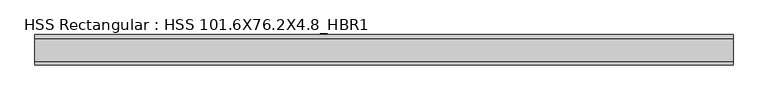
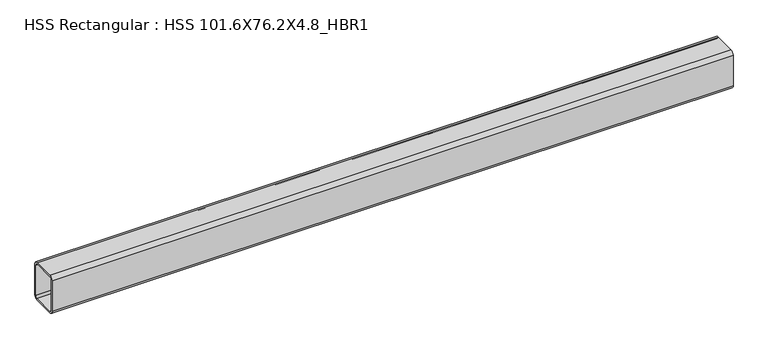
"""IFC4 building model written with IfcOpenShell, lengths in millimetres: beam geometry, HSS Rectangular : HSS 101.6X76.2X4.8_HBR1."""

from ifc_helpers import new_model, si_unit, point, frame, frame_2d, origin, place, context, project, spatial, polyline, circle_curve, trimmed, segment, composite_curve, outline, extrude, source, transform, mapped, element, save


def hss_rectangular_hss_101_6x76_2x4_8_hbr1_9ee25929(model_context):
    return source(origin(), model_context, "Body", "SweptSolid", [
        extrude(outline(composite_curve([segment(polyline([(38.1, 41.275), (38.1, -41.275)]), True, "CONTINUOUS"), segment(trimmed(circle_curve(frame_2d((28.575, -41.275)), 9.525), [point((38.1, -41.275))], [point((28.575, -50.8))], False, "CARTESIAN"), True, "CONTINUOUS"), segment(polyline([(28.575, -50.8), (-28.575, -50.8)]), True, "CONTINUOUS"), segment(trimmed(circle_curve(frame_2d((-28.575, -41.275)), 9.525), [point((-28.575, -50.8))], [point((-38.1, -41.275))], False, "CARTESIAN"), True, "CONTINUOUS"), segment(polyline([(-38.1, -41.275), (-38.1, 41.275)]), True, "CONTINUOUS"), segment(trimmed(circle_curve(frame_2d((-28.575, 41.275)), 9.525), [point((-38.1, 41.275))], [point((-28.575, 50.8))], False, "CARTESIAN"), True, "CONTINUOUS"), segment(polyline([(-28.575, 50.8), (28.575, 50.8)]), True, "CONTINUOUS"), segment(trimmed(circle_curve(frame_2d((28.575, 41.275)), 9.525), [point((28.575, 50.8))], [point((38.1, 41.275))], False, "CARTESIAN"), True, "CONTINUOUS")], self_intersect=False), holes=[composite_curve([segment(trimmed(circle_curve(frame_2d((-28.575, 41.275)), 4.7625), [point((-28.575, 46.0375))], [point((-33.3375, 41.275))], True, "CARTESIAN"), True, "CONTINUOUS"), segment(polyline([(-33.3375, 41.275), (-33.3375, -41.275)]), True, "CONTINUOUS"), segment(trimmed(circle_curve(frame_2d((-28.575, -41.275)), 4.7625), [point((-33.3375, -41.275))], [point((-28.575, -46.0375))], True, "CARTESIAN"), True, "CONTINUOUS"), segment(polyline([(-28.575, -46.0375), (28.575, -46.0375)]), True, "CONTINUOUS"), segment(trimmed(circle_curve(frame_2d((28.575, -41.275)), 4.7625), [point((28.575, -46.0375))], [point((33.3375, -41.275))], True, "CARTESIAN"), True, "CONTINUOUS"), segment(polyline([(33.3375, -41.275), (33.3375, 41.275)]), True, "CONTINUOUS"), segment(trimmed(circle_curve(frame_2d((28.575, 41.275)), 4.7625), [point((33.3375, 41.275))], [point((28.575, 46.0375))], True, "CARTESIAN"), True, "CONTINUOUS"), segment(polyline([(28.575, 46.0375), (-28.575, 46.0375)]), True, "CONTINUOUS")], self_intersect=False)]), frame((-850.0, 0.0, 0.0), z_axis=(1.0, 0.0, 0.0), x_axis=(0.0, 1.0, 0.0)), (0.0, 0.0, 1.0), 1747.4492101),
    ])


if __name__ == "__main__":
    model = new_model("IFC4")
    model_context = context("Model", 3, world=origin())
    ifc_project = project(units=[si_unit("LENGTHUNIT", "METRE", prefix="MILLI")], contexts=[model_context])
    site = spatial("IfcSite", under=ifc_project)
    building = spatial("IfcBuilding", under=site)
    placement = place(None, origin())
    hss_rectangular_hss_101_6x76_2x4_8_hbr1_shape = hss_rectangular_hss_101_6x76_2x4_8_hbr1_9ee25929(model_context)
    element("IfcBeam", 1, ObjectType="HSS Rectangular : HSS 101.6X76.2X4.8_HBR1", at=placement, inside=building, context=model_context, shape_type="MappedRepresentation", body=[
        mapped(hss_rectangular_hss_101_6x76_2x4_8_hbr1_shape, transform((0.0, 0.0, 0.0), x_axis=(1.0, 0.0, 0.0), y_axis=(0.0, 1.0, 0.0), z_axis=(0.0, 0.0, 1.0))),
    ])
    save(model, "model.ifc")

# Revit data of these elements
# Type "HSS Rectangular : HSS 101.6X76.2X4.8_HBR1"
#   Section Name Key = "HSS 4X3X3/16"
#   Assembly Code = "B10"
#   Width = 7.62 cm
#   Wall Nominal Thickness = 0.4763 cm
#   Wall Design Thickness = 0.442 cm
#   Torsional Moment of Inertia = 260.561 cm⁴
#   Torsional Modulus = 61.2876 cm³
#   Section Area = 14.4516 cm²
#   Plastic Modulus weak axis = 40.3122 cm³
#   Plastic Modulus strong axis = 49.1612 cm³
#   Perimeter = 0.881482 m²/m
#   Outer Fillet = 0.9525 cm
#   Nominal Weight = 12.1285 kgf/m
#   Moment of Inertia weak axis = 131.529 cm⁴
#   Moment of Inertia strong axis = 205.202 cm⁴
#   Inner Fillet = 0.4763 cm
#   Height = 10.16 cm
#   Elastic Modulus weak axis = 34.4128 cm³
#   Elastic Modulus strong axis = 40.476 cm³
#   Centroid Vertical = 5.08 cm
#   Centroid Horizontal = 3.81 cm
#   Length [instance default] = 1524 mm
#   Structural Material [instance default] = Steel ASTM A500, Grade B, Rectangular and Square
#   Principal Axes Angle = 0
# Element 1 (IfcBeam, "HSS Rectangular : HSS 101.6X76.2X4.8_HBR1")
#   Structural Material = Steel ASTM A992
#   Materials on its faces: "Steel ASTM A992"
# Materials
#   "Steel ASTM A500, Grade B, Rectangular and Square": class "Metal", colour RGB 199 199 199, transparency 0, Description = "Carbon steel", Cost = 0
#   "Steel ASTM A992": class "Metal", colour RGB 199 199 199, transparency 0, Description = "Structural steel 50ksi", Cost = 0
